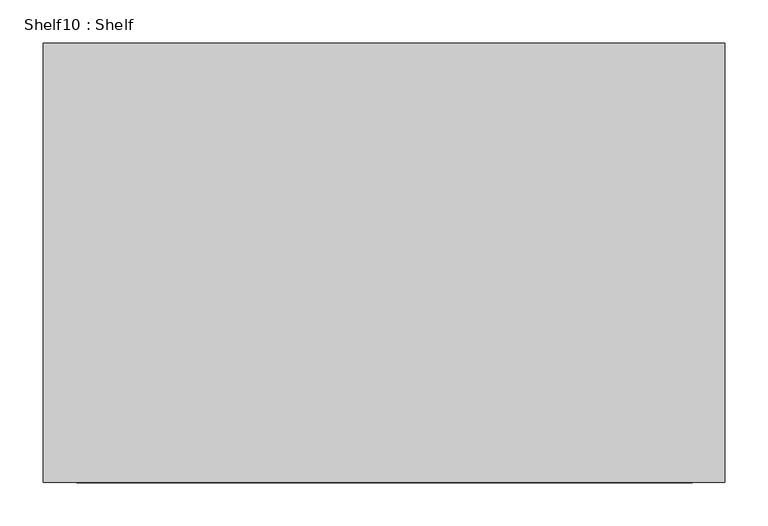
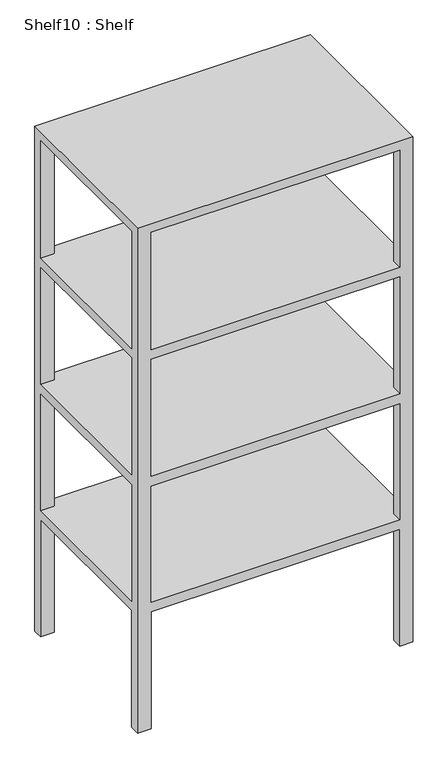
"""IFC4 building model written with IfcOpenShell, lengths in millimetres: furniture geometry, Shelf10 : Shelf."""

from ifc_helpers import new_model, si_unit, origin, place, context, project, spatial, faceted_brep, source, transform, mapped, element, save


def shelf10_shelf_7f4ece80(model_context):
    return source(origin(), model_context, "Body", "Brep", [
        faceted_brep([(14906.8798744, 2223.7615366, 1524.0), (14906.8798744, 2731.7615366, 1524.0), (14119.4798744, 2731.7615366, 1524.0), (14119.4798744, 2223.7615366, 1524.0), (14906.8798744, 2223.7615366, 0.0), (14869.5001442, 2223.7615366, 0.0), (14869.5001442, 2252.7838057, 0.0), (14906.8798744, 2252.7838057, 0.0), (14869.5001442, 2731.7615366, 0.0), (14906.8798744, 2731.7615366, 0.0), (14906.8798744, 2702.8377422, 0.0), (14869.5001442, 2702.8377422, 0.0), (14158.3001442, 2223.7615366, 0.0), (14119.4798744, 2223.7615366, 0.0), (14119.4798744, 2252.7838057, 0.0), (14158.3001442, 2252.7838057, 0.0), (14119.4798744, 2702.8377422, 0.0), (14119.4798744, 2731.7615366, 0.0), (14158.3001442, 2731.7615366, 0.0), (14158.3001442, 2702.8377422, 0.0), (14158.3001442, 2223.7615366, 353.3332002), (14869.5001442, 2223.7615366, 353.3332002), (14158.3001442, 2223.7615366, 1497.6781444), (14869.5001442, 2223.7615366, 1497.6781444), (14869.5001442, 2223.7615366, 1143.0), (14158.3001442, 2223.7615366, 1143.0), (14158.3001442, 2223.7615366, 1114.8196695), (14869.5001442, 2223.7615366, 1114.8196695), (14869.5001442, 2223.7615366, 762.0), (14158.3001442, 2223.7615366, 762.0), (14158.3001442, 2223.7615366, 731.9611947), (14869.5001442, 2223.7615366, 731.9611947), (14869.5001442, 2223.7615366, 381.0), (14158.3001442, 2223.7615366, 381.0), (14119.4798744, 2702.8377422, 353.3332002), (14119.4798744, 2252.7838057, 353.3332002), (14119.4798744, 2702.8377422, 1497.6781444), (14119.4798744, 2252.3559348, 1497.6781444), (14119.4798744, 2252.3559348, 1143.0), (14119.4798744, 2702.8377422, 1143.0), (14119.4798744, 2702.8377422, 1114.8196695), (14119.4798744, 2252.7838057, 1114.8196695), (14119.4798744, 2252.7838057, 762.0), (14119.4798744, 2702.8377422, 762.0), (14119.4798744, 2702.8377422, 731.9611947), (14119.4798744, 2252.7838057, 731.9611947), (14119.4798744, 2252.7838057, 381.0), (14119.4798744, 2702.8377422, 381.0), (14869.5001442, 2731.7615366, 353.3332002), (14158.3001442, 2731.7615366, 353.3332002), (14869.5001442, 2731.7615366, 1497.6781444), (14158.3001442, 2731.7615366, 1497.6781444), (14158.3001442, 2731.7615366, 1143.0), (14869.5001442, 2731.7615366, 1143.0), (14869.5001442, 2731.7615366, 1114.8196695), (14158.3001442, 2731.7615366, 1114.8196695), (14158.3001442, 2731.7615366, 762.0), (14869.5001442, 2731.7615366, 762.0), (14869.5001442, 2731.7615366, 731.9611947), (14158.3001442, 2731.7615366, 731.9611947), (14158.3001442, 2731.7615366, 381.0), (14869.5001442, 2731.7615366, 381.0), (14906.8798744, 2252.7838057, 353.3332002), (14906.8798744, 2702.8377422, 353.3332002), (14906.8798744, 2252.7838057, 1497.6781444), (14906.8798744, 2702.8377422, 1497.6781444), (14906.8798744, 2702.8377422, 1143.0), (14906.8798744, 2252.7838057, 1143.0), (14906.8798744, 2252.7838057, 1114.8196695), (14906.8798744, 2702.8377422, 1114.8196695), (14906.8798744, 2702.8377422, 762.0), (14906.8798744, 2252.7838057, 762.0), (14906.8798744, 2252.7838057, 731.9611947), (14906.8798744, 2702.8377422, 731.9611947), (14906.8798744, 2702.8377422, 381.0), (14906.8798744, 2252.7838057, 381.0), (14158.3001442, 2702.8377422, 1497.6781444), (14869.5001442, 2702.8377422, 1497.6781444), (14869.5001442, 2252.7838057, 1497.6781444), (14158.3001442, 2252.3559348, 1497.6781444), (14158.3001442, 2702.8377422, 1143.0), (14158.3001442, 2252.3559348, 1143.0), (14869.5001442, 2252.7838057, 1143.0), (14869.5001442, 2702.8377422, 1143.0), (14158.3001442, 2702.8377422, 1114.8196695), (14869.5001442, 2702.8377422, 1114.8196695), (14869.5001442, 2252.7838057, 1114.8196695), (14158.3001442, 2252.7838057, 1114.8196695), (14158.3001442, 2702.8377422, 762.0), (14158.3001442, 2252.7838057, 762.0), (14869.5001442, 2252.7838057, 762.0), (14869.5001442, 2702.8377422, 762.0), (14158.3001442, 2702.8377422, 731.9611947), (14869.5001442, 2702.8377422, 731.9611947), (14869.5001442, 2252.7838057, 731.9611947), (14158.3001442, 2252.7838057, 731.9611947), (14158.3001442, 2702.8377422, 381.0), (14158.3001442, 2252.7838057, 381.0), (14869.5001442, 2252.7838057, 381.0), (14869.5001442, 2702.8377422, 381.0), (14158.3001442, 2702.8377422, 353.3332002), (14869.5001442, 2702.8377422, 353.3332002), (14869.5001442, 2252.7838057, 353.3332002), (14158.3001442, 2252.7838057, 353.3332002)], [[[0, 1, 2, 3]], [[4, 5, 6, 7]], [[8, 9, 10, 11]], [[12, 13, 14, 15]], [[16, 17, 18, 19]], [[0, 3, 13, 12, 20, 21, 5, 4], [22, 23, 24, 25], [26, 27, 28, 29], [30, 31, 32, 33]], [[3, 2, 17, 16, 34, 35, 14, 13], [36, 37, 38, 39], [40, 41, 42, 43], [44, 45, 46, 47]], [[2, 1, 9, 8, 48, 49, 18, 17], [50, 51, 52, 53], [54, 55, 56, 57], [58, 59, 60, 61]], [[1, 0, 4, 7, 62, 63, 10, 9], [64, 65, 66, 67], [68, 69, 70, 71], [72, 73, 74, 75]], [[76, 51, 50, 77, 65, 64, 78, 23, 22, 79, 37, 36]], [[80, 39, 38, 81, 25, 24, 82, 67, 66, 83, 53, 52]], [[51, 76, 80, 52]], [[77, 50, 53, 83]], [[65, 77, 83, 66]], [[78, 64, 67, 82]], [[23, 78, 82, 24]], [[79, 22, 25, 81]], [[37, 79, 81, 38]], [[76, 36, 39, 80]], [[84, 55, 54, 85, 69, 68, 86, 27, 26, 87, 41, 40]], [[88, 43, 42, 89, 29, 28, 90, 71, 70, 91, 57, 56]], [[55, 84, 88, 56]], [[85, 54, 57, 91]], [[69, 85, 91, 70]], [[86, 68, 71, 90]], [[27, 86, 90, 28]], [[87, 26, 29, 89]], [[41, 87, 89, 42]], [[84, 40, 43, 88]], [[92, 59, 58, 93, 73, 72, 94, 31, 30, 95, 45, 44]], [[96, 47, 46, 97, 33, 32, 98, 75, 74, 99, 61, 60]], [[59, 92, 96, 60]], [[93, 58, 61, 99]], [[73, 93, 99, 74]], [[94, 72, 75, 98]], [[31, 94, 98, 32]], [[95, 30, 33, 97]], [[45, 95, 97, 46]], [[92, 44, 47, 96]], [[100, 49, 48, 101, 63, 62, 102, 21, 20, 103, 35, 34]], [[49, 100, 19, 18]], [[101, 48, 8, 11]], [[63, 101, 11, 10]], [[102, 62, 7, 6]], [[21, 102, 6, 5]], [[103, 20, 12, 15]], [[35, 103, 15, 14]], [[100, 34, 16, 19]]]),
    ])


if __name__ == "__main__":
    model = new_model("IFC4")
    model_context = context("Model", 3, world=origin())
    ifc_project = project(units=[si_unit("LENGTHUNIT", "METRE", prefix="MILLI")], contexts=[model_context])
    site = spatial("IfcSite", under=ifc_project)
    building = spatial("IfcBuilding", under=site)
    placement = place(None, origin())
    shelf10_shelf_shape = shelf10_shelf_7f4ece80(model_context)
    element("IfcFurniture", 1, ObjectType="Shelf10 : Shelf", at=placement, inside=building, context=model_context, shape_type="MappedRepresentation", body=[
        mapped(shelf10_shelf_shape, transform((0.0, 0.0, 0.0), x_axis=(1.0, 0.0, 0.0), y_axis=(0.0, 1.0, 0.0), z_axis=(0.0, 0.0, 1.0))),
    ])
    save(model, "model.ifc")

# Revit data of these elements
# Element 1 (IfcFurniture, "Shelf10 : Shelf")
#   Materials on its faces: "food"
# Materials
#   "food": class "Glass", colour RGB 233 233 233, transparency 0, Description = "Soda Lime Glass", Cost = 0
